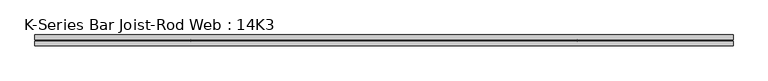
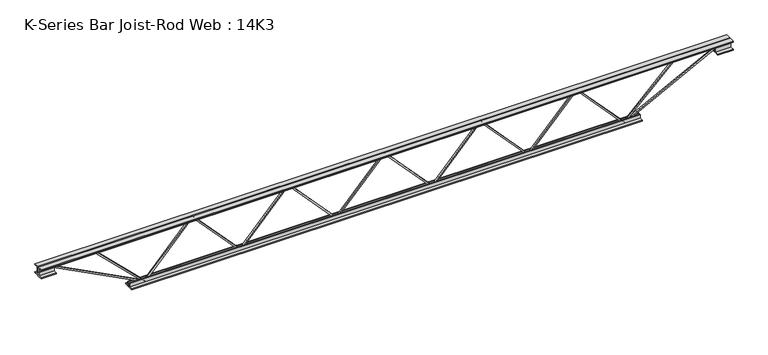
"""IFC4 building model written with IfcOpenShell, lengths in millimetres: beam geometry, K-Series Bar Joist-Rod Web : 14K3."""

from ifc_helpers import new_model, si_unit, frame, origin, place, context, project, spatial, polyline, outline, extrude, source, transform, mapped, element, save


def k_series_bar_joist_rod_web_14k3_1543307f(model_context):
    return source(origin(), model_context, "Body", "SweptSolid", [
        extrude(outline(polyline([(-166.6875, 322.58), (-176.2125, 322.58), (-176.2125, 327.8414815), (166.6875, 644.0714815), (166.6875, 646.2485185), (-176.2125, 962.4785185), (-176.2125, 967.74), (-166.6875, 967.74), (-166.6875, 966.6514815), (176.2125, 650.4214815), (176.2125, 639.8985185), (-166.6875, 323.6685185), (-166.6875, 322.58)])), frame((0.0, -4.7625, 0.0), z_axis=(0.0, 1.0, 0.0), x_axis=(0.0, 0.0, 1.0)), (0.0, 0.0, 1.0), 9.525),
        extrude(outline(polyline([(-166.6875, -322.58), (-176.2125, -322.58), (-176.2125, -317.3185185), (166.6875, -1.0885185), (166.6875, 1.0885185), (-176.2125, 317.3185185), (-176.2125, 322.58), (-166.6875, 322.58), (-166.6875, 321.4914815), (176.2125, 5.2614815), (176.2125, -5.2614815), (-166.6875, -321.4914815), (-166.6875, -322.58)])), frame((0.0, -4.7625, 0.0), z_axis=(0.0, 1.0, 0.0), x_axis=(0.0, 0.0, 1.0)), (0.0, 0.0, 1.0), 9.525),
        extrude(outline(polyline([(-166.6875, -967.74), (-176.2125, -967.74), (-176.2125, -962.4785185), (166.6875, -646.2485185), (166.6875, -644.0714815), (-176.2125, -327.8414815), (-176.2125, -322.58), (-166.6875, -322.58), (-166.6875, -323.6685185), (176.2125, -639.8985185), (176.2125, -650.4214815), (-166.6875, -966.6514815), (-166.6875, -967.74)])), frame((0.0, -4.7625, 0.0), z_axis=(0.0, 1.0, 0.0), x_axis=(0.0, 0.0, 1.0)), (0.0, 0.0, 1.0), 9.525),
        extrude(outline(polyline([(-166.6875, 967.74), (-176.2125, 967.74), (-176.2125, 973.0014815), (166.6875, 1289.2314815), (166.6875, 1291.4085185), (-176.2125, 1607.6385185), (-176.2125, 1612.9), (-166.6875, 1612.9), (-166.6875, 1611.8114815), (176.2125, 1295.5814815), (176.2125, 1285.0585185), (-166.6875, 968.8285185), (-166.6875, 967.74)])), frame((0.0, -4.7625, 0.0), z_axis=(0.0, 1.0, 0.0), x_axis=(0.0, 0.0, 1.0)), (0.0, 0.0, 1.0), 9.525),
        extrude(outline(polyline([(-166.6875, -1612.9), (-176.2125, -1612.9), (-176.2125, -1607.6385185), (166.6875, -1291.4085185), (166.6875, -1289.2314815), (-176.2125, -973.0014815), (-176.2125, -967.74), (-166.6875, -967.74), (-166.6875, -968.8285185), (176.2125, -1285.0585185), (176.2125, -1295.5814815), (-166.6875, -1611.8114815), (-166.6875, -1612.9)])), frame((0.0, -4.7625, 0.0), z_axis=(0.0, 1.0, 0.0), x_axis=(0.0, 0.0, 1.0)), (0.0, 0.0, 1.0), 9.525),
        extrude(outline(polyline([(4.7625, 177.8), (36.5125, 177.8), (36.5125, 171.45), (11.1125, 171.45), (11.1125, 146.05), (4.7625, 146.05), (4.7625, 177.8)])), frame((-2324.1, 0.0, 0.0), z_axis=(1.0, 0.0, 0.0), x_axis=(0.0, 1.0, 0.0)), (0.0, 0.0, 1.0), 4648.2),
        extrude(outline(polyline([(-4.7625, 177.8), (-4.7625, 146.05), (-11.1125, 146.05), (-11.1125, 171.45), (-36.5125, 171.45), (-36.5125, 177.8), (-4.7625, 177.8)])), frame((-2324.1, 0.0, 0.0), z_axis=(1.0, 0.0, 0.0), x_axis=(0.0, 1.0, 0.0)), (0.0, 0.0, 1.0), 4648.2),
        extrude(outline(polyline([(-4.7625, 114.3), (-36.5125, 114.3), (-36.5125, 120.65), (-11.1125, 120.65), (-11.1125, 146.05), (-4.7625, 146.05), (-4.7625, 114.3)])), frame((-2324.1, 0.0, 0.0), z_axis=(1.0, 0.0, 0.0), x_axis=(0.0, 1.0, 0.0)), (0.0, 0.0, 1.0), 101.6),
        extrude(outline(polyline([(36.5125, 114.3), (4.7625, 114.3), (4.7625, 146.05), (11.1125, 146.05), (11.1125, 120.65), (36.5125, 120.65), (36.5125, 114.3)])), frame((-2324.1, 0.0, 0.0), z_axis=(1.0, 0.0, 0.0), x_axis=(0.0, 1.0, 0.0)), (0.0, 0.0, 1.0), 101.6),
        extrude(outline(polyline([(4.7625, 114.3), (4.7625, 146.05), (11.1125, 146.05), (11.1125, 120.65), (36.5125, 120.65), (36.5125, 114.3), (4.7625, 114.3)])), frame((2222.5, 0.0, 0.0), z_axis=(1.0, 0.0, 0.0), x_axis=(0.0, 1.0, 0.0)), (0.0, 0.0, 1.0), 101.6),
        extrude(outline(polyline([(-4.7625, 114.3), (-36.5125, 114.3), (-36.5125, 120.65), (-11.1125, 120.65), (-11.1125, 146.05), (-4.7625, 146.05), (-4.7625, 114.3)])), frame((2222.5, 0.0, 0.0), z_axis=(1.0, 0.0, 0.0), x_axis=(0.0, 1.0, 0.0)), (0.0, 0.0, 1.0), 101.6),
        extrude(outline(polyline([(4.7625, -177.8), (4.7625, -146.05), (11.1125, -146.05), (11.1125, -171.45), (36.5125, -171.45), (36.5125, -177.8), (4.7625, -177.8)])), frame((-1714.5, 0.0, 0.0), z_axis=(1.0, 0.0, 0.0), x_axis=(0.0, 1.0, 0.0)), (0.0, 0.0, 1.0), 3429.0),
        extrude(outline(polyline([(-4.7625, -177.8), (-36.5125, -177.8), (-36.5125, -171.45), (-11.1125, -171.45), (-11.1125, -146.05), (-4.7625, -146.05), (-4.7625, -177.8)])), frame((-1714.5, 0.0, 0.0), z_axis=(1.0, 0.0, 0.0), x_axis=(0.0, 1.0, 0.0)), (0.0, 0.0, 1.0), 3429.0),
        extrude(outline(polyline([(0.0, -9.525), (0.0, 0.0), (687.3270037, 0.0), (687.3270037, -9.525), (0.0, -9.525)])), frame((-2224.6999627, 4.7625, 141.8260717), z_axis=(0.4619344188366021, 0.0, 0.8869140841671704), x_axis=(0.8869140841671704, 0.0, -0.4619344188366021)), (0.0, 0.0, 1.0), 9.525),
        extrude(outline(polyline([(0.0, -9.525), (0.0, 0.0), (452.6191627, 0.0), (452.6191627, -9.525), (0.0, -9.525)])), frame((-1938.8207639, 4.7625, 142.6557839), z_axis=(0.7014727307155686, 0.0, 0.7126962944076835), x_axis=(0.7126962944076835, 0.0, -0.7014727307155686)), (0.0, 0.0, 1.0), 9.525),
        extrude(outline(polyline([(0.0, -9.525), (0.0, 0.0), (687.3270037, 0.0), (687.3270037, -9.525), (0.0, -9.525)])), frame((2224.6999627, -4.7625, 141.8260717), z_axis=(-0.4619344188365845, 0.0, 0.8869140841671797), x_axis=(-0.8869140841671797, 0.0, -0.4619344188365845)), (0.0, 0.0, 1.0), 9.525),
        extrude(outline(polyline([(0.0, -9.525), (0.0, 0.0), (452.6191627, 0.0), (452.6191627, -9.525), (0.0, -9.525)])), frame((1938.8207639, -4.7625, 142.6557839), z_axis=(-0.7014727307155634, 0.0, 0.7126962944076886), x_axis=(-0.7126962944076886, 0.0, -0.7014727307155634)), (0.0, 0.0, 1.0), 9.525),
    ])


if __name__ == "__main__":
    model = new_model("IFC4")
    model_context = context("Model", 3, world=origin())
    ifc_project = project(units=[si_unit("LENGTHUNIT", "METRE", prefix="MILLI")], contexts=[model_context])
    site = spatial("IfcSite", under=ifc_project)
    building = spatial("IfcBuilding", under=site)
    placement = place(None, origin())
    k_series_bar_joist_rod_web_14k3_shape = k_series_bar_joist_rod_web_14k3_1543307f(model_context)
    element("IfcBeam", 1, ObjectType="K-Series Bar Joist-Rod Web : 14K3", at=placement, inside=building, context=model_context, shape_type="MappedRepresentation", body=[
        mapped(k_series_bar_joist_rod_web_14k3_shape, transform((0.0, 0.0, 0.0), x_axis=(1.0, 0.0, 0.0), y_axis=(0.0, 1.0, 0.0), z_axis=(0.0, 0.0, 1.0))),
    ])
    save(model, "model.ifc")

# Revit data of these elements
# Type "K-Series Bar Joist-Rod Web : 14K3"
#   Assembly Code = "B1010350"
#   Wt = 6
#   Web Thickness = 0' - 0 3/8"
#   Start Offset [instance default] = 0' - 0"
#   Start Extension [instance default] = 0' - 0"
#   Seat Length = 0' - 4"
#   Seat Depth = 0' - 2 1/2"
#   PanelArrayLength [instance default] = 19' - 4"
#   Panel [instance default] = 2' - 5"
#   End Offset [instance default] = 0' - 0"
#   End Extension [instance default] = 0' - 0"
#   End Panel = 2' - 4"
#   Cord Leg = 0' - 1 1/4"
#   Chord Thickness = 0' - 0 1/4"
#   Length [instance default] = 24' - 0"
#   Depth = 1' - 2"
#   PanelArrayNum [instance default] = 8
#   Structural Material = none
# Element 1 (IfcBeam, "K-Series Bar Joist-Rod Web : 14K3")
#   PanelArrayLength = 10' - 7"
#   Panel = 2' - 1.4"
#   PanelArrayNum = 5
